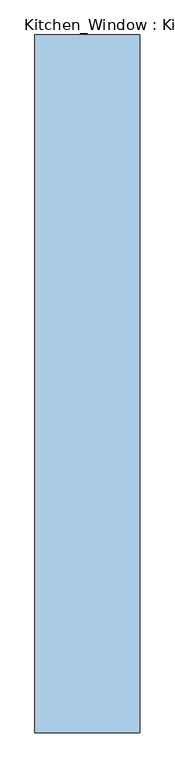
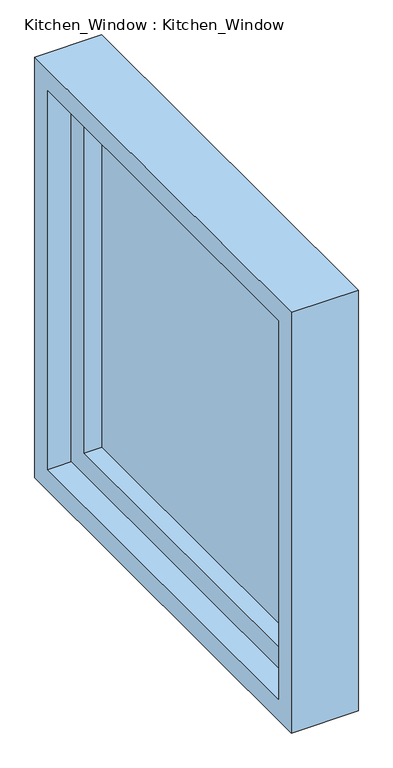
"""IFC4 building model written with IfcOpenShell, lengths in millimetres: window geometry, Kitchen_Window : Kitchen_Window."""

from ifc_helpers import new_model, si_unit, frame, origin, place, context, project, spatial, polyline, outline, extrude, source, transform, mapped, element, save


def kitchen_window_kitchen_window_f07ff302(model_context):
    return source(origin(), model_context, "Body", "SweptSolid", [
        extrude(outline(polyline([(4355.0, 10455.0), (4355.0, 11245.0), (4365.0, 11245.0), (4365.0, 10455.0), (4355.0, 10455.0)])), frame((0.0, 0.0, 1555.0), z_axis=(0.0, 0.0, 1.0), x_axis=(1.0, 0.0, 0.0)), (0.0, 0.0, 1.0), 790.0),
        extrude(outline(polyline([(11295.0, 2395.0), (11295.0, 1505.0), (10405.0, 1505.0), (10405.0, 2395.0), (11295.0, 2395.0)]), holes=[polyline([(11245.0, 1555.0), (11245.0, 2345.0), (10455.0, 2345.0), (10455.0, 1555.0), (11245.0, 1555.0)])]), frame((4315.0, 0.0, 0.0), z_axis=(1.0, 0.0, 0.0), x_axis=(0.0, 1.0, 0.0)), (0.0, 0.0, 1.0), 100.0),
        extrude(outline(polyline([(11350.0, 2450.0), (11350.0, 1450.0), (10350.0, 1450.0), (10350.0, 2450.0), (11350.0, 2450.0)]), holes=[polyline([(11300.0, 1500.0), (11300.0, 2400.0), (10400.0, 2400.0), (10400.0, 1500.0), (11300.0, 1500.0)])]), frame((4265.0, 0.0, 0.0), z_axis=(1.0, 0.0, 0.0), x_axis=(0.0, 1.0, 0.0)), (0.0, 0.0, 1.0), 150.0),
    ])


if __name__ == "__main__":
    model = new_model("IFC4")
    model_context = context("Model", 3, world=origin())
    ifc_project = project(units=[si_unit("LENGTHUNIT", "METRE", prefix="MILLI")], contexts=[model_context])
    site = spatial("IfcSite", under=ifc_project)
    building = spatial("IfcBuilding", under=site)
    placement = place(None, origin())
    kitchen_window_kitchen_window_shape = kitchen_window_kitchen_window_f07ff302(model_context)
    element("IfcWindow", 1, ObjectType="Kitchen_Window : Kitchen_Window", at=placement, inside=building, context=model_context, shape_type="MappedRepresentation", body=[
        mapped(kitchen_window_kitchen_window_shape, transform((0.0, 0.0, 0.0), x_axis=(1.0, 0.0, 0.0), y_axis=(0.0, 1.0, 0.0), z_axis=(0.0, 0.0, 1.0))),
    ])
    save(model, "model.ifc")

# Revit data of these elements
# Type "Kitchen_Window : Kitchen_Window"
#   Type Mark = "53"
#   NameOverride = "Kitchen_Window"
# Element 1 (IfcWindow, "Kitchen_Window : Kitchen_Window")
#   Materials on its faces: "IfcSurfaceStyle #392", "IfcSurfaceStyle #398"
# Materials
#   "IfcSurfaceStyle #392": class "Unassigned", colour RGB 204 204 204, transparency 0
#   "IfcSurfaceStyle #398": class "Unassigned", colour RGB 93 183 203, transparency 0.85
